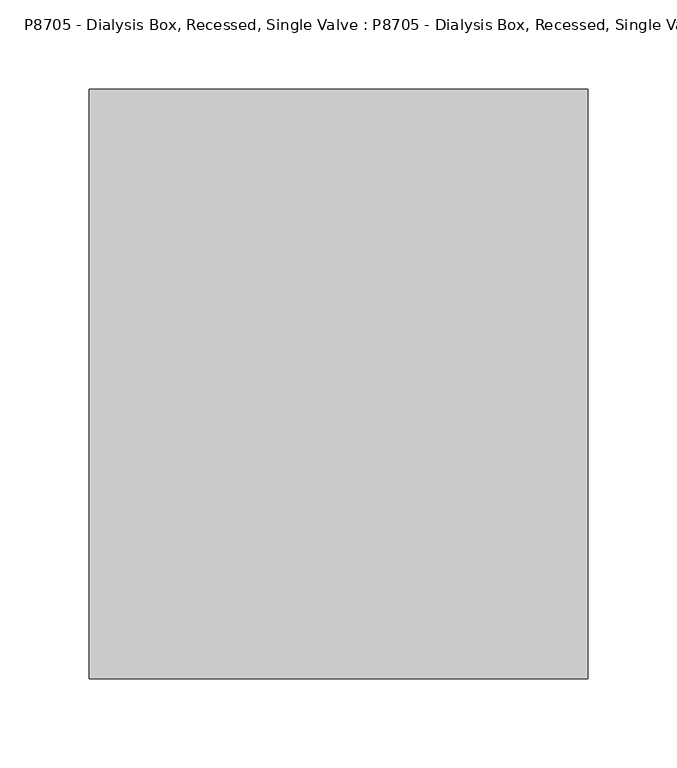
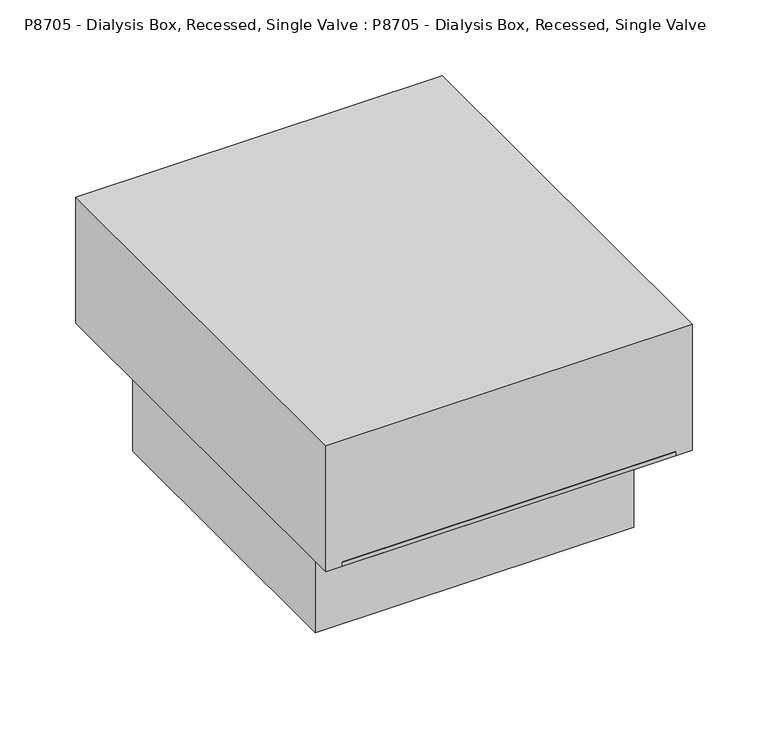
"""IFC4 building model written with IfcOpenShell, lengths in millimetres: proxy geometry, P8705 - Dialysis Box, Recessed, Single Valve : P8705 - Dialysis Box, Recessed, Single Valve."""

import ifcopenshell
import ifcopenshell.guid

model = None  # the IFC model being written
_history = None  # IfcOwnerHistory: only IFC2X3 demands one
_inside = {}  # id of a spatial element -> (the spatial element, [elements in it])
_under = {}  # id of a project, library or spatial element -> (it, [spatial elements below it])
_declared = {}  # id of a project -> (the project, [libraries it declares])
_typed = {}  # id of a type object -> (the type object, [elements of that type])
_made_of = {}  # id of a material, layer set ... -> (it, [elements and type objects made of it])


def new_model(schema):
    """Start an empty IFC model of exactly this schema.

    Asked for "IFC4X3", IfcOpenShell would pick the latest addendum, in which some entities
    have other attributes; the version numbers below select the first issue.
    IFC2X3 requires an IfcOwnerHistory on every rooted entity: one is made here for all.
    """
    global model, _history
    if schema == "IFC4X3":
        model = ifcopenshell.file(schema_version=(4, 3, 0, 0))
    else:
        model = ifcopenshell.file(schema=schema)
    _inside.clear()
    _under.clear()
    _declared.clear()
    _typed.clear()
    _made_of.clear()
    _history = None
    if model.schema == "IFC2X3":
        org = make("IfcOrganization", Name="unknown")
        user = make(
            "IfcPersonAndOrganization",
            ThePerson=make("IfcPerson", FamilyName="unknown"),
            TheOrganization=org,
        )
        app = make(
            "IfcApplication",
            ApplicationDeveloper=org,
            Version="unknown",
            ApplicationFullName="unknown",
            ApplicationIdentifier="unknown",
        )
        _history = make(
            "IfcOwnerHistory",
            OwningUser=user,
            OwningApplication=app,
            ChangeAction="ADDED",
            CreationDate=0,
        )
    return model


def make(cls, **values):
    """One entity of the class cls with the attributes given. An attribute that is None is left unset."""
    return model.create_entity(
        cls, **{name: value for name, value in values.items() if value is not None}
    )


def rooted(cls, **values):
    """An entity with a GlobalId (a new one), such as an element, a storey or a relation."""
    return make(cls, GlobalId=ifcopenshell.guid.new(), OwnerHistory=_history, **values)


def si_unit(unit_type, name, prefix=None):
    """IfcSIUnit, for example si_unit("LENGTHUNIT", "METRE", prefix="MILLI")."""
    return make("IfcSIUnit", UnitType=unit_type, Prefix=prefix, Name=name)


def assignment(units):
    """IfcUnitAssignment: the units of a project."""
    return None if units is None else make("IfcUnitAssignment", Units=units)


def point(xyz):
    """IfcCartesianPoint."""
    return None if xyz is None else make("IfcCartesianPoint", Coordinates=xyz)


def direction(xyz):
    """IfcDirection."""
    return None if xyz is None else make("IfcDirection", DirectionRatios=xyz)


def frame(location, z_axis=None, x_axis=None):
    """IfcAxis2Placement3D, a coordinate frame: its origin and axes. An axis left out is left unset."""
    return make(
        "IfcAxis2Placement3D",
        Location=point(location),
        Axis=direction(z_axis),
        RefDirection=direction(x_axis),
    )


def origin():
    """The frame at (0, 0, 0) with its axes left unset."""
    return frame((0.0, 0.0, 0.0))


def origin_with_axes():
    """The frame at (0, 0, 0) with the z axis (0, 0, 1) and the x axis (1, 0, 0) written out."""
    return frame((0.0, 0.0, 0.0), z_axis=(0.0, 0.0, 1.0), x_axis=(1.0, 0.0, 0.0))


def place(relative_to, where):
    """IfcLocalPlacement: puts the frame where relative to a parent placement (None: the world)."""
    return make(
        "IfcLocalPlacement", PlacementRelTo=relative_to, RelativePlacement=where
    )


def context(
    kind, dimensions, precision=None, world=None, true_north=None, identifier=None
):
    """IfcGeometricRepresentationContext, for example the 3D "Model" context."""
    return make(
        "IfcGeometricRepresentationContext",
        ContextIdentifier=identifier,
        ContextType=kind,
        CoordinateSpaceDimension=dimensions,
        Precision=precision,
        WorldCoordinateSystem=world,
        TrueNorth=true_north,
    )


def project(units=None, contexts=None):
    """IfcProject with its units and contexts."""
    return rooted(
        "IfcProject",
        Name="project",
        RepresentationContexts=contexts,
        UnitsInContext=assignment(units),
    )


def spatial(cls, under=None, at=None, **own):
    """A site, building, storey or space (cls), placed at a placement, below another one or the project."""
    s = rooted(cls, ObjectPlacement=at, **own)
    if under is not None:
        _under.setdefault(under.id(), (under, []))[1].append(s)
    return s


def polyline(points):
    """IfcPolyline through the points."""
    return make("IfcPolyline", Points=[point(p) for p in points])


def outline(outer, holes=None, kind="AREA"):
    """IfcArbitraryClosedProfileDef: a profile drawn as a closed curve; with holes, ...WithVoids."""
    if holes is None:
        return make("IfcArbitraryClosedProfileDef", ProfileType=kind, OuterCurve=outer)
    return make(
        "IfcArbitraryProfileDefWithVoids",
        ProfileType=kind,
        OuterCurve=outer,
        InnerCurves=holes,
    )


def extrude(swept, where, along, depth):
    """IfcExtrudedAreaSolid: the profile swept, set in the frame where, extruded along a direction by depth."""
    return make(
        "IfcExtrudedAreaSolid",
        SweptArea=swept,
        Position=where,
        ExtrudedDirection=direction(along),
        Depth=depth,
    )


def faces_of(points, faces, orient=None, outer=None):
    """IfcFace entities. A face is a list of loops; a loop is a list of indices into points, from 0.

    orient and outer hold one flag for each loop. By default every Orientation is true, the
    first loop of a face is its IfcFaceOuterBound and the others are IfcFaceBound.
    """
    made = []
    for i, loops in enumerate(faces):
        bounds = []
        for j, loop in enumerate(loops):
            is_outer = j == 0 if outer is None else outer[i][j]
            bounds.append(
                make(
                    "IfcFaceOuterBound" if is_outer else "IfcFaceBound",
                    Bound=make("IfcPolyLoop", Polygon=[points[k] for k in loop]),
                    Orientation=True if orient is None else orient[i][j],
                )
            )
        made.append(make("IfcFace", Bounds=bounds))
    return made


def faceted_brep(points, faces, orient=None, outer=None, voids=None):
    """IfcFacetedBrep: a solid bounded by flat faces; with voids (closed shells), ...WithVoids."""
    shared = [point(p) for p in points]
    hull = make("IfcClosedShell", CfsFaces=faces_of(shared, faces, orient, outer))
    if voids is None:
        return make("IfcFacetedBrep", Outer=hull)
    return make(
        "IfcFacetedBrepWithVoids",
        Outer=hull,
        Voids=[
            make(cls, CfsFaces=faces_of(shared, fs, o, b)) for cls, fs, o, b in voids
        ],
    )


def shape(context_of_items, identifier, shape_type, items):
    """IfcShapeRepresentation: the items that make up one representation, for example the "Body"."""
    return make(
        "IfcShapeRepresentation",
        ContextOfItems=context_of_items,
        RepresentationIdentifier=identifier,
        RepresentationType=shape_type,
        Items=items,
    )


def source(mapping_origin, context_of_items, identifier, shape_type, items):
    """IfcRepresentationMap: a shape defined once, which mapped items show again and again."""
    return make(
        "IfcRepresentationMap",
        MappingOrigin=mapping_origin,
        MappedRepresentation=shape(context_of_items, identifier, shape_type, items),
    )


def transform(
    local_origin,
    x_axis=None,
    y_axis=None,
    z_axis=None,
    scale=None,
    scale2=None,
    scale3=None,
    uniform=True,
):
    """IfcCartesianTransformationOperator3D, or its non-uniform kind. x_axis, y_axis, z_axis: its Axis1, 2, 3."""
    if uniform:
        return make(
            "IfcCartesianTransformationOperator3D",
            Axis1=direction(x_axis),
            Axis2=direction(y_axis),
            LocalOrigin=point(local_origin),
            Scale=scale,
            Axis3=direction(z_axis),
        )
    return make(
        "IfcCartesianTransformationOperator3DnonUniform",
        Axis1=direction(x_axis),
        Axis2=direction(y_axis),
        LocalOrigin=point(local_origin),
        Scale=scale,
        Axis3=direction(z_axis),
        Scale2=scale2,
        Scale3=scale3,
    )


def mapped(mapping_source, mapping_target):
    """IfcMappedItem: shows the shape of a source again, moved by a transform."""
    return make(
        "IfcMappedItem", MappingSource=mapping_source, MappingTarget=mapping_target
    )


def made_of(thing, what):
    """Note that an element or type object is made of a material, layer set ...; save() writes the relation."""
    if what is not None:
        _made_of.setdefault(what.id(), (what, []))[1].append(thing)
    return thing


def element(
    cls,
    number,
    at=None,
    inside=None,
    cuts=None,
    type_object=None,
    material=None,
    context=None,
    identifier="Body",
    shape_type=None,
    held_by="IfcProductDefinitionShape",
    body=None,
    shapes=None,
    **own,
):
    """One element of the class cls, such as IfcWall. Its Tag is "e" and its number.

    at: its placement. inside: the storey or other place that contains it. cuts: it is an
    opening in that element (IfcRelVoidsElement). A single representation is given by context,
    identifier, shape_type and body (its items); several are given by shapes. held_by: the class
    of the entity that holds the representations. save() writes the other relations.
    """
    e = rooted(cls, Tag="e%d" % number, ObjectPlacement=at, **own)
    if body is not None:
        shapes = [shape(context, identifier, shape_type, body)]
    if shapes is not None:
        e.Representation = make(held_by, Representations=shapes)
    if inside is not None:
        _inside.setdefault(inside.id(), (inside, []))[1].append(e)
    if cuts is not None:
        rooted(
            "IfcRelVoidsElement", RelatingBuildingElement=cuts, RelatedOpeningElement=e
        )
    if type_object is not None:
        _typed.setdefault(type_object.id(), (type_object, []))[1].append(e)
    return made_of(e, material)


def aggregate(whole, parts):
    """IfcRelAggregates: a whole, such as a stair, and the parts it consists of."""
    return rooted("IfcRelAggregates", RelatingObject=whole, RelatedObjects=parts)


def save(model, path):
    """Write the relations noted so far, then the file.

    IfcRelAggregates (storeys below a building ...), IfcRelContainedInSpatialStructure (elements
    in a storey), IfcRelDefinesByType, IfcRelAssociatesMaterial and IfcRelDeclares: one each for
    every whole, place, type object, material and project.
    """
    for whole, parts in _under.values():
        aggregate(whole, parts)
    for where, things in _inside.values():
        rooted(
            "IfcRelContainedInSpatialStructure",
            RelatedElements=things,
            RelatingStructure=where,
        )
    for kind, things in _typed.values():
        rooted("IfcRelDefinesByType", RelatedObjects=things, RelatingType=kind)
    for what, things in _made_of.values():
        rooted("IfcRelAssociatesMaterial", RelatedObjects=things, RelatingMaterial=what)
    for by, libraries in _declared.values():
        rooted("IfcRelDeclares", RelatingContext=by, RelatedDefinitions=libraries)
    model.write(path)


def p8705_dialysis_box_recessed_single_valve_p8705_dialysis_box_98d03597(model_context):
    return source(origin(), model_context, "Body", "SolidModel", [
        faceted_brep([(127.0, -165.1, 3.175), (127.0, 165.1, 3.175), (-127.0, 165.1, 3.175), (-127.0, -165.1, 3.175), (114.3, 101.6, 3.175), (114.3, -101.9737484, 3.175), (-114.3, -101.9737484, 3.175), (-114.3, 101.6, 3.175), (127.0, -165.1, 0.0), (-127.0, -165.1, 0.0), (-127.0, 165.1, 0.0), (127.0, 165.1, 0.0), (120.65, 120.65, 0.0), (-122.0738096, 120.65, 0.0), (-122.0738096, -120.65, 0.0), (120.65, -120.65, 0.0), (120.65, -120.65, -82.55), (120.65, 120.65, -82.55), (-122.0738096, 120.65, -82.55), (-122.0738096, -120.65, -82.55), (-114.3, 101.6, -76.2), (114.3, 101.6, -76.2), (114.3, -101.9737484, -76.2), (-114.3, -101.9737484, -76.2)], [[[0, 1, 2, 3], [4, 5, 6, 7]], [[8, 9, 10, 11], [12, 13, 14, 15]], [[3, 9, 8, 0]], [[2, 10, 9, 3]], [[1, 11, 10, 2]], [[0, 8, 11, 1]], [[12, 15, 16, 17]], [[14, 13, 18, 19]], [[17, 18, 13, 12]], [[16, 19, 18, 17]], [[15, 14, 19, 16]], [[4, 7, 20, 21]], [[6, 5, 22, 23]], [[7, 6, 23, 20]], [[20, 23, 22, 21]], [[21, 22, 5, 4]]]),
        extrude(outline(polyline([(139.7, -165.1), (-139.7, -165.1), (-139.7, 165.1), (139.7, 165.1), (139.7, -165.1)])), origin_with_axes(), (0.0, 0.0, 1.0), 101.6),
    ])


if __name__ == "__main__":
    model = new_model("IFC4")
    model_context = context("Model", 3, world=origin())
    ifc_project = project(units=[si_unit("LENGTHUNIT", "METRE", prefix="MILLI")], contexts=[model_context])
    site = spatial("IfcSite", under=ifc_project)
    building = spatial("IfcBuilding", under=site)
    placement = place(None, origin())
    p8705_dialysis_box_recessed_single_valve_p8705_dialysis_box_shape = p8705_dialysis_box_recessed_single_valve_p8705_dialysis_box_98d03597(model_context)
    element("IfcBuildingElementProxy", 1, Name="P8705 - Dialysis Box, Recessed, Single Valve : P8705 - Dialysis Box, Recessed, Single Valve", ObjectType="P8705 - Dialysis Box, Recessed, Single Valve : P8705 - Dialysis Box, Recessed, Single Valve", at=placement, inside=building, context=model_context, shape_type="MappedRepresentation", body=[
        mapped(p8705_dialysis_box_recessed_single_valve_p8705_dialysis_box_shape, transform((0.0, 0.0, 0.0), x_axis=(1.0, 0.0, 0.0), y_axis=(0.0, 1.0, 0.0), z_axis=(0.0, 0.0, 1.0))),
    ])
    save(model, "model.ifc")

# Revit data of these elements
# Type "P8705 - Dialysis Box, Recessed, Single Valve : P8705 - Dialysis Box, Recessed, Single Valve"
#   Watts2 = "0"
#   Watts1 = "0"
#   Unit_Issue = "EA"
#   UTIL_6_Misc = "-"
#   UTIL_5_NonMedGas = "-"
#   UTIL_4_MiscGas = "-"
#   UTIL_3_MedGas = "-"
#   UTIL_2_Elec = "-"
#   UTIL_1_WaterDrain = "B"
#   Nomenclature = "Dialysis Box, Recessed, Single Valve"
#   NSN = "4100"
#   Location [instance default] = ""
#   JSN = "P8705"
#   Fund_Source_VA = "-"
#   Fund_Source_Navy = "-"
#   Fund_Source_Army = "-"
#   Fund_Source_AF = "-"
#   ELEC_Volts2 = "0"
#   ELEC_Volts1 = "0"
#   ELEC_Phase2 = "0"
#   ELEC_Phase1 = "0"
#   ELEC_HertzSwitch = "0"
#   ELEC_HertzDependent = "0"
#   ELEC_Hertz = "0"
#   ELEC_Amps2 = "0"
#   ELEC_Amps1 = "0"
#   DetailDescription = "A single cold water valve supply, recessed dialysis box with door. Box is constructed of stainless steel and includes the following standard equipment: cold water valve with 1/2\" nom. copper female inlet, 3/4\" male hose thread outlet and vacuum breaker; discharge hose bracket, waste water receptor, and removable wall flange. For use only in the ICU and other acute areas when a patient cannot be moved to the dialysis unit."
#   CAT_VA = "A"
#   CAT_Navy = "A"
#   CAT_IHS = "-"
#   CAT_Army = "A"
#   CAT_AF = "A"
#   BTUperhour = "0"
#   Weight_IP = 5
#   Default Elevation = 4' - 6"
#   DIM_Width_IP = 0' - 11"
#   DIM_Height_IP = 1' - 1"
#   DIM_Depth_IP = 0' - 4"
#   Assembly Code = ""
# Element 1 (IfcBuildingElementProxy, "P8705 - Dialysis Box, Recessed, Single Valve : P8705 - Dialysis Box, Recessed, Single Valve")
#   Materials on its faces: "Finish", "EquipSpace"
# Materials
#   "Finish": class "Plastic", colour RGB 245 239 218, transparency 0
#   "EquipSpace": class "Unassigned", colour RGB 221 217 195, transparency 0.5
